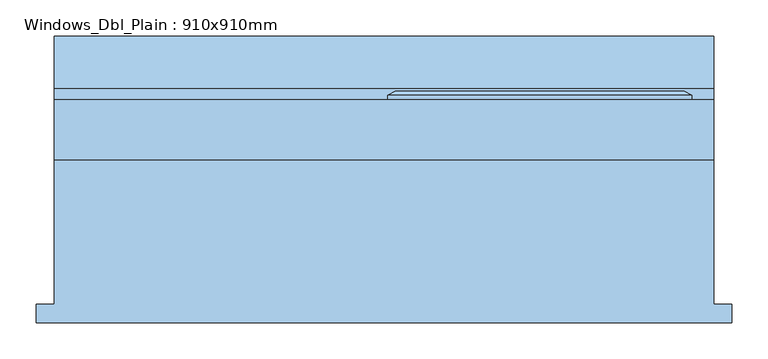
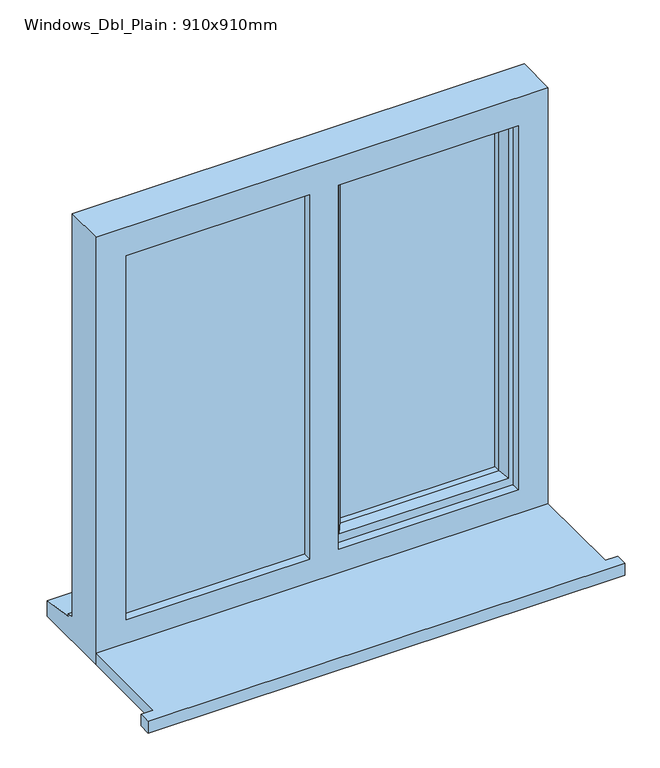
"""IFC4 building model written with IfcOpenShell, lengths in millimetres: window geometry, Windows_Dbl_Plain : 910x910mm."""

from ifc_helpers import new_model, si_unit, frame, origin, place, context, project, spatial, polyline, outline, extrude, faceted_brep, source, transform, mapped, element, save


def windows_dbl_plain_910x910mm_1b1950ab(model_context):
    return source(origin(), model_context, "Body", "SolidModel", [
        extrude(outline(polyline([(-765.0, -182.7934322), (-765.0, -157.7934322), (-740.0, -157.7934322), (-740.0, 41.7065678), (170.0, 41.7065678), (170.0, -157.7934322), (195.0, -157.7934322), (195.0, -182.7934322), (-765.0, -182.7934322)])), frame((0.0, 0.0, 1200.0), z_axis=(0.0, 0.0, 1.0), x_axis=(1.0, 0.0, 0.0)), (0.0, 0.0, 1.0), 25.0),
        extrude(outline(polyline([(100.0, 88.7065678), (-240.0, 88.7065678), (-240.0, 112.7065678), (100.0, 112.7065678), (100.0, 88.7065678)])), frame((0.0, 0.0, 1293.0), z_axis=(0.0, 0.0, 1.0), x_axis=(1.0, 0.0, 0.0)), (0.0, 0.0, 1.0), 747.0),
        extrude(outline(polyline([(-700.0, 83.7065678), (-300.0, 83.7065678), (-300.0, 59.7065678), (-700.0, 59.7065678), (-700.0, 83.7065678)])), frame((0.0, 0.0, 1263.0), z_axis=(0.0, 0.0, 1.0), x_axis=(1.0, 0.0, 0.0)), (0.0, 0.0, 1.0), 807.0),
        faceted_brep([(170.0, 41.7065678, 2110.0), (-740.0, 41.7065678, 2110.0), (-740.0, 41.7065678, 1200.0), (170.0, 41.7065678, 1200.0), (110.0, 41.7065678, 2050.0), (110.0, 41.7065678, 1275.0), (-252.0, 41.7065678, 1275.0), (-252.0, 41.7065678, 2050.0), (-310.0, 41.7065678, 2050.0), (-310.0, 41.7065678, 1275.0), (-680.0, 41.7065678, 1275.0), (-680.0, 41.7065678, 2050.0), (-740.0, 124.7065678, 2110.0), (-740.0, 124.7065678, 1251.0), (-740.0, 139.7065678, 1249.68767), (-740.0, 139.7065678, 1244.7449676), (-740.0, 212.2065678, 1233.8088847), (-740.0, 212.2065678, 1200.0), (170.0, 124.7065678, 2110.0), (170.0, 124.7065678, 1251.0), (-700.0, 124.7065678, 2070.0), (-700.0, 124.7065678, 1263.0), (-310.0, 124.7065678, 1263.0), (-310.0, 124.7065678, 2070.0), (-270.0, 124.7065678, 2070.0), (-270.0, 124.7065678, 1263.0), (130.0, 124.7065678, 1263.0), (130.0, 124.7065678, 2070.0), (-700.0, 59.7065678, 2070.0), (-700.0, 59.7065678, 1263.0), (-300.0, 59.7065678, 2070.0), (-300.0, 59.7065678, 1263.0), (-310.0, 59.7065678, 2050.0), (-680.0, 59.7065678, 2050.0), (-680.0, 59.7065678, 1275.0), (-310.0, 59.7065678, 1275.0), (-270.0, 59.7065678, 2070.0), (130.0, 59.7065678, 2070.0), (130.0, 59.7065678, 1263.0), (-270.0, 59.7065678, 1263.0), (110.0, 59.7065678, 2050.0), (-252.0, 59.7065678, 2050.0), (-252.0, 59.7065678, 1275.0), (110.0, 59.7065678, 1275.0), (-310.0, 83.7065678, 2070.0), (-300.0, 83.7065678, 2070.0), (170.0, 212.2065678, 1200.0), (170.0, 212.2065678, 1233.8088847), (170.0, 139.7065678, 1244.7449676), (170.0, 139.7065678, 1249.68767), (-300.0, 83.7065678, 1263.0), (-310.0, 83.7065678, 1263.0)], [[[0, 1, 2, 3], [4, 5, 6, 7], [8, 9, 10, 11]], [[2, 1, 12, 13, 14, 15, 16, 17]], [[13, 12, 18, 19], [20, 21, 22, 23], [24, 25, 26, 27]], [[21, 20, 28, 29]], [[28, 30, 31, 29], [32, 33, 34, 35]], [[36, 37, 38, 39], [40, 41, 42, 43]], [[33, 11, 10, 34]], [[1, 0, 18, 12]], [[28, 20, 23, 44, 45, 30]], [[27, 37, 36, 24]], [[11, 33, 32, 8]], [[40, 4, 7, 41]], [[19, 18, 0, 3, 46, 47, 48, 49]], [[27, 26, 38, 37]], [[4, 40, 43, 5]], [[45, 50, 31, 30]], [[50, 45, 44, 51]], [[51, 44, 23, 22]], [[25, 24, 36, 39]], [[41, 7, 6, 42]], [[8, 32, 35, 9]], [[46, 3, 2, 17]], [[47, 46, 17, 16]], [[48, 47, 16, 15]], [[49, 48, 15, 14]], [[19, 49, 14, 13]], [[22, 21, 29, 31, 50, 51]], [[26, 25, 39, 38]], [[6, 5, 43, 42]], [[35, 34, 10, 9]]]),
        extrude(outline(polyline([(2050.0, -310.0), (2070.0, -310.0), (2070.0, -700.0), (1263.0, -700.0), (1263.0, -310.0), (1283.0, -310.0), (1283.0, -680.0), (2050.0, -680.0), (2050.0, -310.0)])), frame((0.0, 83.7065678, 0.0), z_axis=(0.0, 1.0, 0.0), x_axis=(0.0, 0.0, 1.0)), (0.0, 0.0, 1.0), 41.0),
        faceted_brep([(-280.0, 124.7065678, 2080.0), (-280.0, 130.4800705, 2080.0), (-280.0, 130.4800705, 1253.0), (-280.0, 124.7065678, 1253.0), (-270.0, 59.7065678, 2070.0), (-270.0, 124.7065678, 2070.0), (-270.0, 124.7065678, 1263.0), (-270.0, 59.7065678, 1263.0), (-230.0, 74.1994677, 2030.0), (-240.1480377, 59.7065678, 2040.1480377), (-240.1480377, 59.7065678, 1292.8519623), (-230.0, 74.1994677, 1303.0), (-230.0, 88.7065678, 2030.0), (-230.0, 88.7065678, 1303.0), (-240.0, 112.7065678, 2040.0), (-240.0, 88.7065678, 2040.0), (-240.0, 88.7065678, 1293.0), (-240.0, 112.7065678, 1293.0), (-230.0, 130.4800705, 2030.0), (-230.0, 112.7065678, 2030.0), (-230.0, 112.7065678, 1303.0), (-230.0, 130.4800705, 1303.0), (-247.4457548, 136.2535732, 2047.4457548), (-247.4457548, 136.2535732, 1285.5542452), (-269.2153903, 136.2535732, 2069.2153903), (-269.2153903, 136.2535732, 1263.7846097), (140.0, 130.4800705, 1253.0), (140.0, 124.7065678, 1253.0), (130.0, 124.7065678, 1263.0), (130.0, 59.7065678, 1263.0), (100.1480377, 59.7065678, 1292.8519623), (90.0, 74.1994677, 1303.0), (90.0, 88.7065678, 1303.0), (100.0, 88.7065678, 1293.0), (100.0, 112.7065678, 1293.0), (90.0, 112.7065678, 1303.0), (90.0, 130.4800705, 1303.0), (107.4457548, 136.2535732, 1285.5542452), (129.2153903, 136.2535732, 1263.7846097), (140.0, 130.4800705, 2080.0), (140.0, 124.7065678, 2080.0), (130.0, 124.7065678, 2070.0), (130.0, 59.7065678, 2070.0), (100.1480377, 59.7065678, 2040.1480377), (90.0, 74.1994677, 2030.0), (90.0, 88.7065678, 2030.0), (100.0, 88.7065678, 2040.0), (100.0, 112.7065678, 2040.0), (90.0, 112.7065678, 2030.0), (90.0, 130.4800705, 2030.0), (107.4457548, 136.2535732, 2047.4457548), (129.2153903, 136.2535732, 2069.2153903)], [[[0, 1, 2, 3]], [[4, 5, 6, 7]], [[8, 9, 10, 11]], [[12, 8, 11, 13]], [[14, 15, 16, 17]], [[18, 19, 20, 21]], [[22, 18, 21, 23]], [[1, 24, 25, 2]], [[3, 2, 26, 27]], [[7, 6, 28, 29]], [[11, 10, 30, 31]], [[13, 11, 31, 32]], [[17, 16, 33, 34]], [[21, 20, 35, 36]], [[23, 21, 36, 37]], [[2, 25, 38, 26]], [[27, 26, 39, 40]], [[29, 28, 41, 42]], [[31, 30, 43, 44]], [[32, 31, 44, 45]], [[34, 33, 46, 47]], [[36, 35, 48, 49]], [[37, 36, 49, 50]], [[26, 38, 51, 39]], [[40, 39, 1, 0]], [[3, 27, 40, 0], [5, 41, 28, 6]], [[42, 41, 5, 4]], [[7, 29, 42, 4], [9, 43, 30, 10]], [[44, 43, 9, 8]], [[45, 44, 8, 12]], [[15, 46, 33, 16], [13, 32, 45, 12]], [[47, 46, 15, 14]], [[17, 34, 47, 14], [19, 48, 35, 20]], [[49, 48, 19, 18]], [[50, 49, 18, 22]], [[24, 51, 38, 25], [23, 37, 50, 22]], [[39, 51, 24, 1]]]),
    ])


if __name__ == "__main__":
    model = new_model("IFC4")
    model_context = context("Model", 3, world=origin())
    ifc_project = project(units=[si_unit("LENGTHUNIT", "METRE", prefix="MILLI")], contexts=[model_context])
    site = spatial("IfcSite", under=ifc_project)
    building = spatial("IfcBuilding", under=site)
    placement = place(None, origin())
    windows_dbl_plain_910x910mm_shape = windows_dbl_plain_910x910mm_1b1950ab(model_context)
    element("IfcWindow", 1, ObjectType="Windows_Dbl_Plain : 910x910mm", at=placement, inside=building, context=model_context, shape_type="MappedRepresentation", body=[
        mapped(windows_dbl_plain_910x910mm_shape, transform((0.0, 0.0, 0.0), x_axis=(1.0, 0.0, 0.0), y_axis=(0.0, 1.0, 0.0), z_axis=(0.0, 0.0, 1.0))),
    ])
    save(model, "model.ifc")

# Revit data of these elements
# Type "Windows_Dbl_Plain : 910x910mm"
#   Type Mark = "80"
#   Operation = "DoublePanelVertical"
#   Construction Type Id = "GSP4R"
#   Manufacturer = "Revit"
#   Keynote = "L10"
#   Analytic Construction = "1/8 in Pilkington single glazing"
#   Wrap Layers (Ext) from Ext = 102.5 mm
#   Wrap Layers (Int) from Ext = 177.5 mm
#   Window Board Projection = 25 mm
#   Window Board Extension = 25 mm
#   Visual Light Transmittance = 0.9
#   Solar Heat Gain Coefficient = 0.78
#   Rough Width = 910 mm
#   Rough Height = 910 mm
#   Height = 910 mm
#   Width = 910 mm
#   Heat Transfer Coefficient (U) = 3.6886 W/(m²·K)
#   Glazing Thickness = 24 mm
#   FrameOffset - External = 50 mm
#   Frame Depth = 65 mm
#   Default Head Height = 2110 mm
#   Cill Depth = 87.5 mm
#   Cavity Closer Width = 50 mm
#   Cavity Closer Offset from Ext = 102.5 mm
#   Cavity Closer Depth = 85 mm
#   Vis - Cavity Closers = yes
#   Define Thermal Properties by = 1
#   Material Trim = Window Frame
#   Material Glass = Glass
#   Material Frame = Window Frame
#   Wall Closure = (empty or 0)
# Element 1 (IfcWindow, "Windows_Dbl_Plain : 910x910mm")
#   Materials on its faces: "Window Frame", "Glass"
# Materials
#   "Window Frame": class "Miscellaneous", colour RGB 249 249 249, transparency 0, Keynote = "L10"
#   "Glass": class "Glass", colour RGB 0 128 192, transparency 0.9, Description = "Soda Lime Glass", Cost = 0
